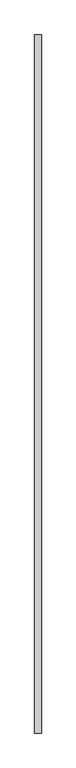
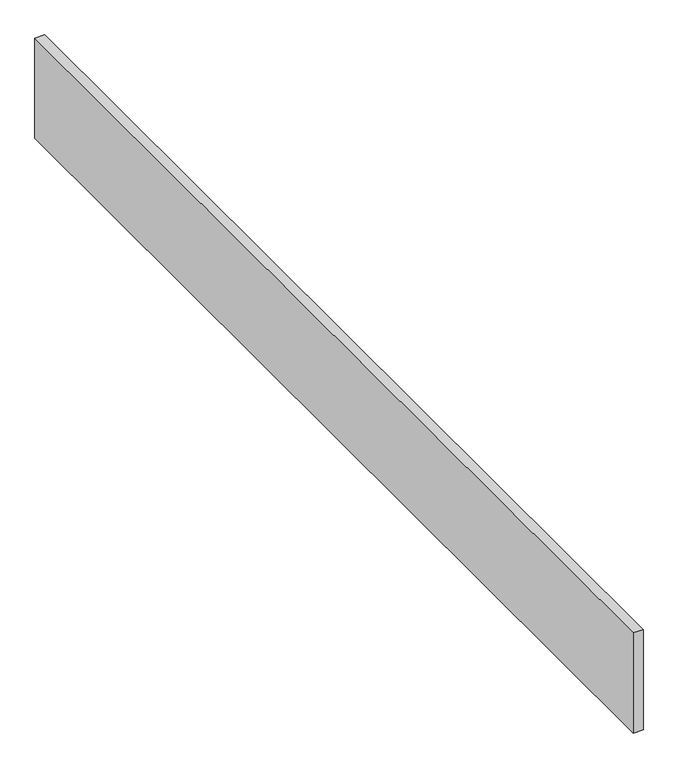
"""IFC4 building model written with IfcOpenShell, lengths in millimetres: proxy geometry, Footer 2604 : Footer 2604."""

from ifc_helpers import new_model, si_unit, frame, origin, place, context, project, spatial, polyline, outline, extrude, source, transform, mapped, element, save


def generic_models_f3d7cf88(model_context):
    return source(origin(), model_context, "Body", "SweptSolid", [
        extrude(outline(polyline([(-931.3315411, -1052.8906574), (-950.3815411, -1052.8906574), (-950.3815411, 947.1093426), (-931.3315411, 947.1093426), (-931.3315411, -1052.8906574)])), frame((0.0, 0.0, 40131.746), z_axis=(0.0, 0.0, 1.0), x_axis=(1.0, 0.0, 0.0)), (0.0, 0.0, 1.0), 204.0961875),
    ])


if __name__ == "__main__":
    model = new_model("IFC4")
    model_context = context("Model", 3, world=origin())
    ifc_project = project(units=[si_unit("LENGTHUNIT", "METRE", prefix="MILLI")], contexts=[model_context])
    site = spatial("IfcSite", under=ifc_project)
    building = spatial("IfcBuilding", under=site)
    placement = place(None, origin())
    generic_models_shape = generic_models_f3d7cf88(model_context)
    element("IfcBuildingElementProxy", 1, Name="Footer 2604 : Footer 2604", ObjectType="Footer 2604 : Footer 2604", at=placement, inside=building, context=model_context, shape_type="MappedRepresentation", body=[
        mapped(generic_models_shape, transform((0.0, 0.0, 0.0), x_axis=(1.0, 0.0, 0.0), y_axis=(0.0, 1.0, 0.0), z_axis=(0.0, 0.0, 1.0))),
    ])
    save(model, "model.ifc")

# Revit data of these elements
# Type "Footer 2604 : Footer 2604"
#   NameOverride = "Footer"
# Element 1 (IfcBuildingElementProxy, "Footer 2604 : Footer 2604")
#   Materials on its faces: "5/8\" GYPSUM BOARD"
# Materials
#   "5/8\" GYPSUM BOARD": class "Unassigned", colour RGB 255 255 255, transparency 0, Cost = 0
